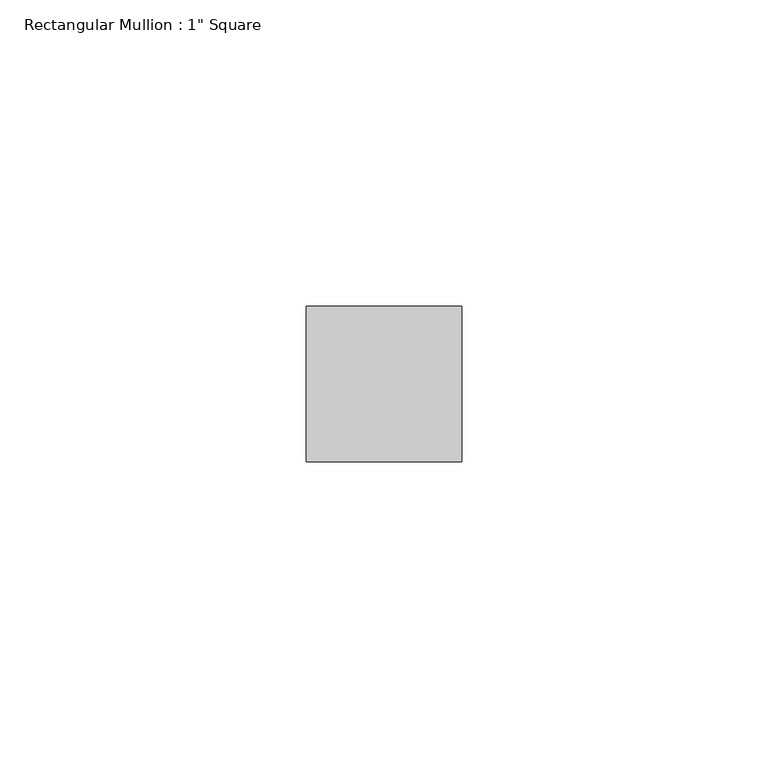
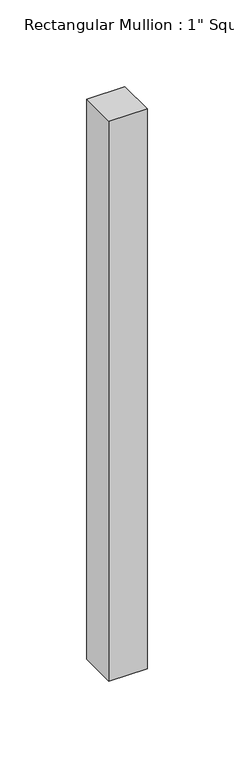
"""IFC4 building model written with IfcOpenShell, lengths in millimetres: member geometry."""

import ifcopenshell
import ifcopenshell.guid

model = None  # the IFC model being written
_history = None  # IfcOwnerHistory: only IFC2X3 demands one
_inside = {}  # id of a spatial element -> (the spatial element, [elements in it])
_under = {}  # id of a project, library or spatial element -> (it, [spatial elements below it])
_declared = {}  # id of a project -> (the project, [libraries it declares])
_typed = {}  # id of a type object -> (the type object, [elements of that type])
_made_of = {}  # id of a material, layer set ... -> (it, [elements and type objects made of it])


def new_model(schema):
    """Start an empty IFC model of exactly this schema.

    Asked for "IFC4X3", IfcOpenShell would pick the latest addendum, in which some entities
    have other attributes; the version numbers below select the first issue.
    IFC2X3 requires an IfcOwnerHistory on every rooted entity: one is made here for all.
    """
    global model, _history
    if schema == "IFC4X3":
        model = ifcopenshell.file(schema_version=(4, 3, 0, 0))
    else:
        model = ifcopenshell.file(schema=schema)
    _inside.clear()
    _under.clear()
    _declared.clear()
    _typed.clear()
    _made_of.clear()
    _history = None
    if model.schema == "IFC2X3":
        org = make("IfcOrganization", Name="unknown")
        user = make(
            "IfcPersonAndOrganization",
            ThePerson=make("IfcPerson", FamilyName="unknown"),
            TheOrganization=org,
        )
        app = make(
            "IfcApplication",
            ApplicationDeveloper=org,
            Version="unknown",
            ApplicationFullName="unknown",
            ApplicationIdentifier="unknown",
        )
        _history = make(
            "IfcOwnerHistory",
            OwningUser=user,
            OwningApplication=app,
            ChangeAction="ADDED",
            CreationDate=0,
        )
    return model


def make(cls, **values):
    """One entity of the class cls with the attributes given. An attribute that is None is left unset."""
    return model.create_entity(
        cls, **{name: value for name, value in values.items() if value is not None}
    )


def rooted(cls, **values):
    """An entity with a GlobalId (a new one), such as an element, a storey or a relation."""
    return make(cls, GlobalId=ifcopenshell.guid.new(), OwnerHistory=_history, **values)


def si_unit(unit_type, name, prefix=None):
    """IfcSIUnit, for example si_unit("LENGTHUNIT", "METRE", prefix="MILLI")."""
    return make("IfcSIUnit", UnitType=unit_type, Prefix=prefix, Name=name)


def assignment(units):
    """IfcUnitAssignment: the units of a project."""
    return None if units is None else make("IfcUnitAssignment", Units=units)


def point(xyz):
    """IfcCartesianPoint."""
    return None if xyz is None else make("IfcCartesianPoint", Coordinates=xyz)


def direction(xyz):
    """IfcDirection."""
    return None if xyz is None else make("IfcDirection", DirectionRatios=xyz)


def frame(location, z_axis=None, x_axis=None):
    """IfcAxis2Placement3D, a coordinate frame: its origin and axes. An axis left out is left unset."""
    return make(
        "IfcAxis2Placement3D",
        Location=point(location),
        Axis=direction(z_axis),
        RefDirection=direction(x_axis),
    )


def origin():
    """The frame at (0, 0, 0) with its axes left unset."""
    return frame((0.0, 0.0, 0.0))


def place(relative_to, where):
    """IfcLocalPlacement: puts the frame where relative to a parent placement (None: the world)."""
    return make(
        "IfcLocalPlacement", PlacementRelTo=relative_to, RelativePlacement=where
    )


def context(
    kind, dimensions, precision=None, world=None, true_north=None, identifier=None
):
    """IfcGeometricRepresentationContext, for example the 3D "Model" context."""
    return make(
        "IfcGeometricRepresentationContext",
        ContextIdentifier=identifier,
        ContextType=kind,
        CoordinateSpaceDimension=dimensions,
        Precision=precision,
        WorldCoordinateSystem=world,
        TrueNorth=true_north,
    )


def project(units=None, contexts=None):
    """IfcProject with its units and contexts."""
    return rooted(
        "IfcProject",
        Name="project",
        RepresentationContexts=contexts,
        UnitsInContext=assignment(units),
    )


def spatial(cls, under=None, at=None, **own):
    """A site, building, storey or space (cls), placed at a placement, below another one or the project."""
    s = rooted(cls, ObjectPlacement=at, **own)
    if under is not None:
        _under.setdefault(under.id(), (under, []))[1].append(s)
    return s


def polyline(points):
    """IfcPolyline through the points."""
    return make("IfcPolyline", Points=[point(p) for p in points])


def outline(outer, holes=None, kind="AREA"):
    """IfcArbitraryClosedProfileDef: a profile drawn as a closed curve; with holes, ...WithVoids."""
    if holes is None:
        return make("IfcArbitraryClosedProfileDef", ProfileType=kind, OuterCurve=outer)
    return make(
        "IfcArbitraryProfileDefWithVoids",
        ProfileType=kind,
        OuterCurve=outer,
        InnerCurves=holes,
    )


def extrude(swept, where, along, depth):
    """IfcExtrudedAreaSolid: the profile swept, set in the frame where, extruded along a direction by depth."""
    return make(
        "IfcExtrudedAreaSolid",
        SweptArea=swept,
        Position=where,
        ExtrudedDirection=direction(along),
        Depth=depth,
    )


def shape(context_of_items, identifier, shape_type, items):
    """IfcShapeRepresentation: the items that make up one representation, for example the "Body"."""
    return make(
        "IfcShapeRepresentation",
        ContextOfItems=context_of_items,
        RepresentationIdentifier=identifier,
        RepresentationType=shape_type,
        Items=items,
    )


def source(mapping_origin, context_of_items, identifier, shape_type, items):
    """IfcRepresentationMap: a shape defined once, which mapped items show again and again."""
    return make(
        "IfcRepresentationMap",
        MappingOrigin=mapping_origin,
        MappedRepresentation=shape(context_of_items, identifier, shape_type, items),
    )


def transform(
    local_origin,
    x_axis=None,
    y_axis=None,
    z_axis=None,
    scale=None,
    scale2=None,
    scale3=None,
    uniform=True,
):
    """IfcCartesianTransformationOperator3D, or its non-uniform kind. x_axis, y_axis, z_axis: its Axis1, 2, 3."""
    if uniform:
        return make(
            "IfcCartesianTransformationOperator3D",
            Axis1=direction(x_axis),
            Axis2=direction(y_axis),
            LocalOrigin=point(local_origin),
            Scale=scale,
            Axis3=direction(z_axis),
        )
    return make(
        "IfcCartesianTransformationOperator3DnonUniform",
        Axis1=direction(x_axis),
        Axis2=direction(y_axis),
        LocalOrigin=point(local_origin),
        Scale=scale,
        Axis3=direction(z_axis),
        Scale2=scale2,
        Scale3=scale3,
    )


def mapped(mapping_source, mapping_target):
    """IfcMappedItem: shows the shape of a source again, moved by a transform."""
    return make(
        "IfcMappedItem", MappingSource=mapping_source, MappingTarget=mapping_target
    )


def made_of(thing, what):
    """Note that an element or type object is made of a material, layer set ...; save() writes the relation."""
    if what is not None:
        _made_of.setdefault(what.id(), (what, []))[1].append(thing)
    return thing


def element(
    cls,
    number,
    at=None,
    inside=None,
    cuts=None,
    type_object=None,
    material=None,
    context=None,
    identifier="Body",
    shape_type=None,
    held_by="IfcProductDefinitionShape",
    body=None,
    shapes=None,
    **own,
):
    """One element of the class cls, such as IfcWall. Its Tag is "e" and its number.

    at: its placement. inside: the storey or other place that contains it. cuts: it is an
    opening in that element (IfcRelVoidsElement). A single representation is given by context,
    identifier, shape_type and body (its items); several are given by shapes. held_by: the class
    of the entity that holds the representations. save() writes the other relations.
    """
    e = rooted(cls, Tag="e%d" % number, ObjectPlacement=at, **own)
    if body is not None:
        shapes = [shape(context, identifier, shape_type, body)]
    if shapes is not None:
        e.Representation = make(held_by, Representations=shapes)
    if inside is not None:
        _inside.setdefault(inside.id(), (inside, []))[1].append(e)
    if cuts is not None:
        rooted(
            "IfcRelVoidsElement", RelatingBuildingElement=cuts, RelatedOpeningElement=e
        )
    if type_object is not None:
        _typed.setdefault(type_object.id(), (type_object, []))[1].append(e)
    return made_of(e, material)


def aggregate(whole, parts):
    """IfcRelAggregates: a whole, such as a stair, and the parts it consists of."""
    return rooted("IfcRelAggregates", RelatingObject=whole, RelatedObjects=parts)


def save(model, path):
    """Write the relations noted so far, then the file.

    IfcRelAggregates (storeys below a building ...), IfcRelContainedInSpatialStructure (elements
    in a storey), IfcRelDefinesByType, IfcRelAssociatesMaterial and IfcRelDeclares: one each for
    every whole, place, type object, material and project.
    """
    for whole, parts in _under.values():
        aggregate(whole, parts)
    for where, things in _inside.values():
        rooted(
            "IfcRelContainedInSpatialStructure",
            RelatedElements=things,
            RelatingStructure=where,
        )
    for kind, things in _typed.values():
        rooted("IfcRelDefinesByType", RelatedObjects=things, RelatingType=kind)
    for what, things in _made_of.values():
        rooted("IfcRelAssociatesMaterial", RelatedObjects=things, RelatingMaterial=what)
    for by, libraries in _declared.values():
        rooted("IfcRelDeclares", RelatingContext=by, RelatedDefinitions=libraries)
    model.write(path)


def member_52f9da16(model_context):
    return source(origin(), model_context, "Body", "SweptSolid", [
        extrude(outline(polyline([(12.7, 12.7), (12.7, -12.7), (-12.7, -12.7), (-12.7, 12.7), (12.7, 12.7)])), frame((0.0, 0.0, -393.7), z_axis=(0.0, 0.0, 1.0), x_axis=(1.0, 0.0, 0.0)), (0.0, 0.0, 1.0), 393.7),
    ])


if __name__ == "__main__":
    model = new_model("IFC4")
    model_context = context("Model", 3, world=origin())
    ifc_project = project(units=[si_unit("LENGTHUNIT", "METRE", prefix="MILLI")], contexts=[model_context])
    site = spatial("IfcSite", under=ifc_project)
    building = spatial("IfcBuilding", under=site)
    placement = place(None, origin())
    member_shape = member_52f9da16(model_context)
    element("IfcMember", 1, ObjectType="Rectangular Mullion : 1\" Square", at=placement, inside=building, context=model_context, shape_type="MappedRepresentation", body=[
        mapped(member_shape, transform((0.0, 0.0, 0.0), x_axis=(1.0, 0.0, 0.0), y_axis=(0.0, 1.0, 0.0), z_axis=(0.0, 0.0, 1.0))),
    ])
    save(model, "model.ifc")

# Revit data of these elements
# Type "Rectangular Mullion : 1\" Square"
#   built-in parameter 1007304 = 0.0833333 (stored number, unit not read)
#   built-in parameter 1007301 = 0.0416667 (stored number, unit not read)
#   built-in parameter 1007300 = 0.0416667 (stored number, unit not read)
# Element 1 (IfcMember, "Rectangular Mullion : 1\" Square")
#   Materials on its faces: "Metal - Aluminum"
# Materials
#   "Metal - Aluminum": class "Metal", colour RGB 247 247 247, transparency 0
